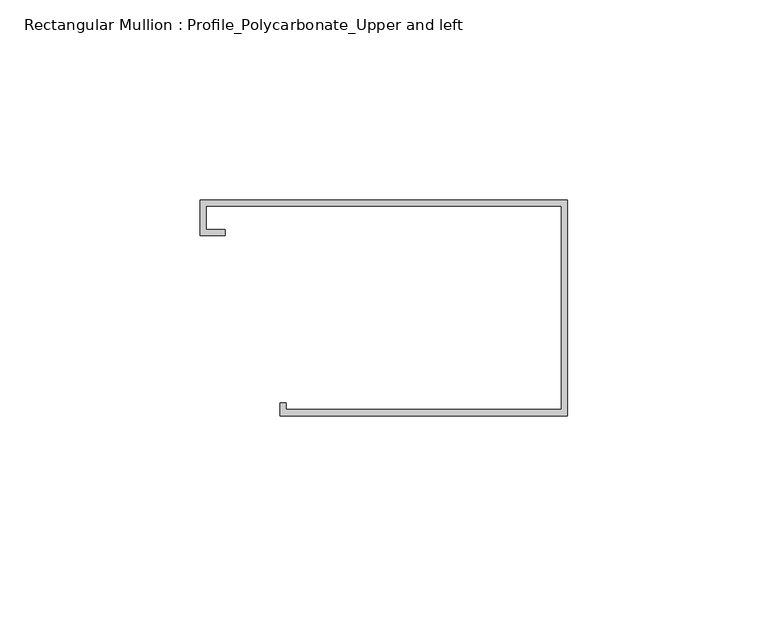
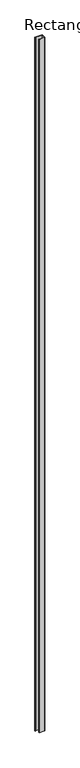
"""IFC4 building model written with IfcOpenShell, lengths in millimetres: member geometry, Rectangular Mullion : Profile_Polycarbonate_Upper and left."""

from ifc_helpers import new_model, si_unit, frame, origin, place, context, project, spatial, polyline, outline, extrude, source, transform, mapped, element, save


def rectangular_mullion_profile_polycarbonate_upper_and_left_ae53e369(model_context):
    return source(origin(), model_context, "Body", "SweptSolid", [
        extrude(outline(polyline([(0.0, 28.984575), (0.0, -25.015825), (-71.9836, -25.015825), (-71.9836, -21.840825), (-70.3961, -21.840825), (-70.3961, -23.428325), (-1.5875, -23.428325), (-1.5875, 27.397075), (-90.4113, 27.397075), (-90.4113, 21.580475), (-85.6488, 21.580475), (-85.6488, 19.992975), (-91.9988, 19.992975), (-91.9988, 28.984575), (0.0, 28.984575)])), frame((0.0, 0.0, -9144.1524), z_axis=(0.0, 0.0, 1.0), x_axis=(1.0, 0.0, 0.0)), (0.0, 0.0, 1.0), 9144.1524),
    ])


if __name__ == "__main__":
    model = new_model("IFC4")
    model_context = context("Model", 3, world=origin())
    ifc_project = project(units=[si_unit("LENGTHUNIT", "METRE", prefix="MILLI")], contexts=[model_context])
    site = spatial("IfcSite", under=ifc_project)
    building = spatial("IfcBuilding", under=site)
    placement = place(None, origin())
    rectangular_mullion_profile_polycarbonate_upper_and_left_shape = rectangular_mullion_profile_polycarbonate_upper_and_left_ae53e369(model_context)
    element("IfcMember", 1, ObjectType="Rectangular Mullion : Profile_Polycarbonate_Upper and left", at=placement, inside=building, context=model_context, shape_type="MappedRepresentation", body=[
        mapped(rectangular_mullion_profile_polycarbonate_upper_and_left_shape, transform((0.0, 0.0, 0.0), x_axis=(1.0, 0.0, 0.0), y_axis=(0.0, 1.0, 0.0), z_axis=(0.0, 0.0, 1.0))),
    ])
    save(model, "model.ifc")

# Revit data of these elements
# Type "Rectangular Mullion : Profile_Polycarbonate_Upper and left"
#   built-in parameter 1007322 = 0.177167 (stored number, unit not read)
#   built-in parameter 1007321 = 0.00520833 (stored number, unit not read)
#   built-in parameter 1007320 = 0 (stored number, unit not read)
